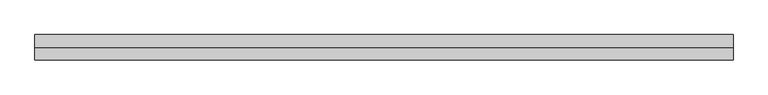
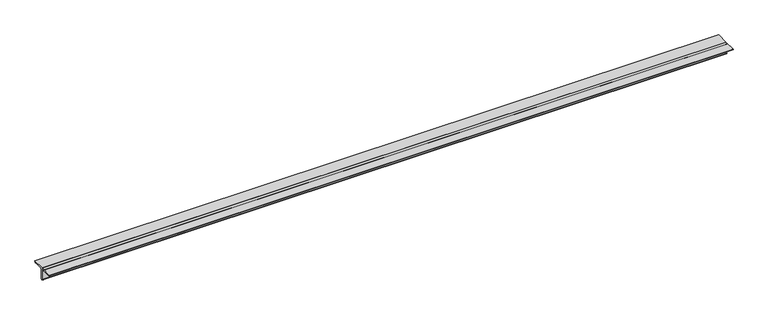
"""IFC4 building model written with IfcOpenShell, lengths in millimetres: member geometry, Steel Framing_2Ls_KS : H_SB_AR_S02_2Ls-100x100x10_VBR1."""

from ifc_helpers import new_model, si_unit, point, frame, frame_2d, origin, place, context, project, spatial, polyline, circle_curve, trimmed, segment, composite_curve, outline, extrude, source, transform, mapped, element, save


def member_76091d96(model_context):
    return source(origin(), model_context, "Body", "SweptSolid", [
        extrude(outline(composite_curve([segment(polyline([(0.0, 28.2), (100.0, 28.2)]), True, "CONTINUOUS"), segment(trimmed(circle_curve(frame_2d((90.0, 28.2)), 10.0), [point((100.0, 28.2))], [point((90.0, 18.2))], False, "CARTESIAN"), True, "CONTINUOUS"), segment(polyline([(90.0, 18.2), (20.0, 18.2)]), True, "CONTINUOUS"), segment(trimmed(circle_curve(frame_2d((20.0, 8.2)), 10.0), [point((20.0, 18.2))], [point((10.0, 8.2))], True, "CARTESIAN"), True, "CONTINUOUS"), segment(polyline([(10.0, 8.2), (10.0, -61.8)]), True, "CONTINUOUS"), segment(trimmed(circle_curve(frame_2d((0.0, -61.8)), 10.0), [point((10.0, -61.8))], [point((0.0, -71.8))], False, "CARTESIAN"), True, "CONTINUOUS"), segment(polyline([(0.0, -71.8), (0.0, 28.2)]), True, "CONTINUOUS")], self_intersect=False)), frame((-2634.5127122, 0.0, 0.0), z_axis=(1.0, 0.0, 0.0), x_axis=(0.0, 1.0, 0.0)), (0.0, 0.0, 1.0), 5511.902449),
        extrude(outline(composite_curve([segment(polyline([(0.0, 28.2), (0.0, -71.8)]), True, "CONTINUOUS"), segment(trimmed(circle_curve(frame_2d((0.0, -61.8)), 10.0), [point((0.0, -71.8))], [point((-10.0, -61.8))], False, "CARTESIAN"), True, "CONTINUOUS"), segment(polyline([(-10.0, -61.8), (-10.0, 8.2)]), True, "CONTINUOUS"), segment(trimmed(circle_curve(frame_2d((-20.0, 8.2)), 10.0), [point((-10.0, 8.2))], [point((-20.0, 18.2))], True, "CARTESIAN"), True, "CONTINUOUS"), segment(polyline([(-20.0, 18.2), (-90.0, 18.2)]), True, "CONTINUOUS"), segment(trimmed(circle_curve(frame_2d((-90.0, 28.2)), 10.0), [point((-90.0, 18.2))], [point((-100.0, 28.2))], False, "CARTESIAN"), True, "CONTINUOUS"), segment(polyline([(-100.0, 28.2), (0.0, 28.2)]), True, "CONTINUOUS")], self_intersect=False)), frame((-2634.5127122, 0.0, 0.0), z_axis=(1.0, 0.0, 0.0), x_axis=(0.0, 1.0, 0.0)), (0.0, 0.0, 1.0), 5511.902449),
    ])


if __name__ == "__main__":
    model = new_model("IFC4")
    model_context = context("Model", 3, world=origin())
    ifc_project = project(units=[si_unit("LENGTHUNIT", "METRE", prefix="MILLI")], contexts=[model_context])
    site = spatial("IfcSite", under=ifc_project)
    building = spatial("IfcBuilding", under=site)
    placement = place(None, origin())
    member_shape = member_76091d96(model_context)
    element("IfcMember", 1, ObjectType="Steel Framing_2Ls_KS : H_SB_AR_S02_2Ls-100x100x10_VBR1", at=placement, inside=building, context=model_context, shape_type="MappedRepresentation", body=[
        mapped(member_shape, transform((0.0, 0.0, 0.0), x_axis=(1.0, 0.0, 0.0), y_axis=(0.0, 1.0, 0.0), z_axis=(0.0, 0.0, 1.0))),
    ])
    save(model, "model.ifc")

# Revit data of these elements
# Type "Steel Framing_2Ls_KS : H_SB_AR_S02_2Ls-100x100x10_VBR1"
#   Type Comments = "MAIN"
#   Type Mark = "VBR1"
#   H_SectionID = "2Ls-100x100x10"
#   Assembly Code = "B10"
#   Legs = "LLBB"
#   H_Ratio for Additional Steel Plate = 0.2
#   W = 0
#   Perimeter = 0.80 m²/m
#   Nominal Weight = 29.80 kgf/m
#   Length [instance default] = 1524 mm
#   Space = 0 mm
#   b = 100 mm
#   d = 100 mm
#   t = 10 mm
#   y = 28.2 mm
#   A = 0.0038 m²
#   Structural Material [instance default] = Steel, 45-345
# Element 1 (IfcMember, "Steel Framing_2Ls_KS : H_SB_AR_S02_2Ls-100x100x10_VBR1")
#   Materials on its faces: "Steel, 45-345"
# Materials
#   "Steel, 45-345": class "Metal", colour RGB 189 187 185, transparency 0, Description = "Steel 345 MPa", Cost = 0
